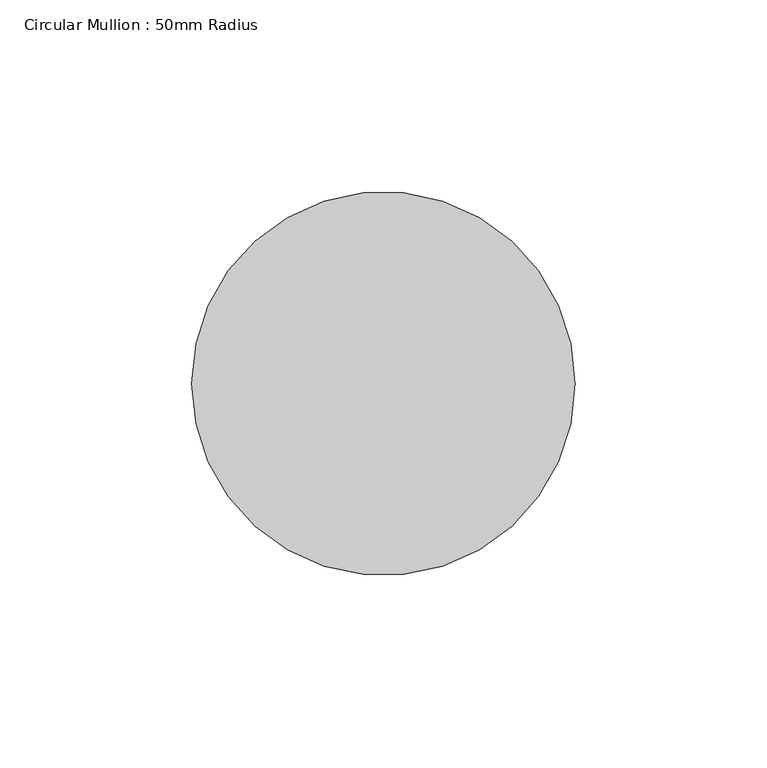
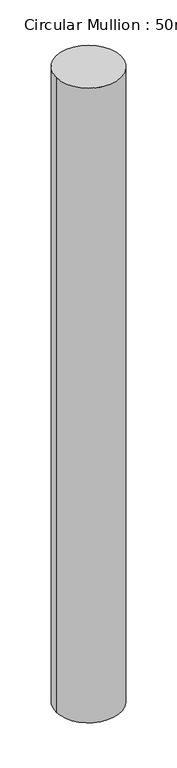
"""IFC4 building model written with IfcOpenShell, lengths in millimetres: member geometry, Circular Mullion : 50mm Radius."""

from ifc_helpers import new_model, si_unit, point, frame, origin, origin_2d, place, context, project, spatial, circle_curve, trimmed, segment, composite_curve, outline, extrude, source, transform, mapped, element, save


def circular_mullion_50mm_radius_80fb73c2(model_context):
    return source(origin(), model_context, "Body", "SweptSolid", [
        extrude(outline(composite_curve([segment(trimmed(circle_curve(origin_2d(), 50.0), [point((50.0, 0.0))], [point((-50.0, 0.0))], False, "CARTESIAN"), True, "CONTINUOUS"), segment(trimmed(circle_curve(origin_2d(), 50.0), [point((-50.0, 0.0))], [point((50.0, 0.0))], False, "CARTESIAN"), True, "CONTINUOUS")], self_intersect=False)), frame((0.0, 0.0, -1035.6265903), z_axis=(0.0, 0.0, 1.0), x_axis=(1.0, 0.0, 0.0)), (0.0, 0.0, 1.0), 1035.6265903),
    ])


if __name__ == "__main__":
    model = new_model("IFC4")
    model_context = context("Model", 3, world=origin())
    ifc_project = project(units=[si_unit("LENGTHUNIT", "METRE", prefix="MILLI")], contexts=[model_context])
    site = spatial("IfcSite", under=ifc_project)
    building = spatial("IfcBuilding", under=site)
    placement = place(None, origin())
    circular_mullion_50mm_radius_shape = circular_mullion_50mm_radius_80fb73c2(model_context)
    element("IfcMember", 1, ObjectType="Circular Mullion : 50mm Radius", at=placement, inside=building, context=model_context, shape_type="MappedRepresentation", body=[
        mapped(circular_mullion_50mm_radius_shape, transform((0.0, 0.0, 0.0), x_axis=(1.0, 0.0, 0.0), y_axis=(0.0, 1.0, 0.0), z_axis=(0.0, 0.0, 1.0))),
    ])
    save(model, "model.ifc")

# Revit data of these elements
# Type "Circular Mullion : 50mm Radius"
#   built-in parameter 1007350 = 0.164042 (stored number, unit not read)
# Element 1 (IfcMember, "Circular Mullion : 50mm Radius")
#   Materials on its faces: "Aluminium"
# Materials
#   "Aluminium": class "Metal", colour RGB 247 247 247, transparency 0, Description = "Aluminium 6061", Cost = 0
